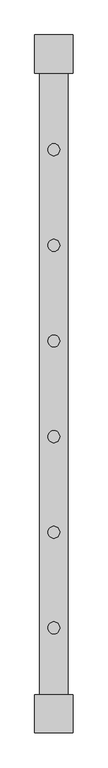
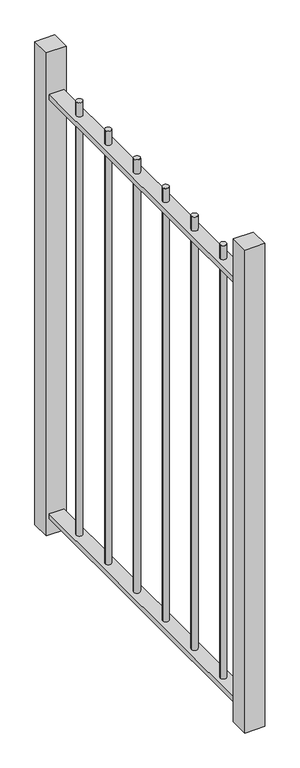
"""IFC4 building model written with IfcOpenShell, lengths in millimetres: railing geometry."""

from ifc_helpers import new_model, si_unit, point, frame, frame_2d, origin, place, context, project, spatial, polyline, circle_curve, trimmed, segment, composite_curve, outline, extrude, source, transform, mapped, element, save


def railing_e03dd60d(model_context):
    return source(origin(), model_context, "Body", "SweptSolid", [
        extrude(outline(polyline([(-6549.419961, 43748.8880881), (-6489.419961, 43748.8880881), (-6489.419961, 42369.1713717), (-6549.419961, 42369.1713717), (-6549.419961, 43748.8880881)])), frame((0.0, 0.0, -30.0), z_axis=(0.0, 0.0, 1.0), x_axis=(1.0, 0.0, 0.0)), (0.0, 0.0, 1.0), 20.0),
        extrude(outline(polyline([(-6549.419961, 43748.8880881), (-6489.419961, 43748.8880881), (-6489.419961, 42369.1713717), (-6549.419961, 42369.1713717), (-6549.419961, 43748.8880881)])), frame((0.0, 0.0, 1750.0), z_axis=(0.0, 0.0, 1.0), x_axis=(1.0, 0.0, 0.0)), (0.0, 0.0, 1.0), 20.0),
        extrude(outline(composite_curve([segment(trimmed(circle_curve(frame_2d((-6519.419961, 42548.8880881)), 12.5), [point((-6531.919961, 42548.8880881))], [point((-6506.919961, 42548.8880881))], False, "CARTESIAN"), True, "CONTINUOUS"), segment(trimmed(circle_curve(frame_2d((-6519.419961, 42548.8880881)), 12.5), [point((-6506.919961, 42548.8880881))], [point((-6531.919961, 42548.8880881))], False, "CARTESIAN"), True, "CONTINUOUS")], self_intersect=False)), frame((0.0, 0.0, -10.0), z_axis=(0.0, 0.0, 1.0), x_axis=(1.0, 0.0, 0.0)), (0.0, 0.0, 1.0), 1840.0),
        extrude(outline(composite_curve([segment(trimmed(circle_curve(frame_2d((-6519.419961, 42748.8880881)), 12.5), [point((-6531.919961, 42748.8880881))], [point((-6506.919961, 42748.8880881))], False, "CARTESIAN"), True, "CONTINUOUS"), segment(trimmed(circle_curve(frame_2d((-6519.419961, 42748.8880881)), 12.5), [point((-6506.919961, 42748.8880881))], [point((-6531.919961, 42748.8880881))], False, "CARTESIAN"), True, "CONTINUOUS")], self_intersect=False)), frame((0.0, 0.0, -10.0), z_axis=(0.0, 0.0, 1.0), x_axis=(1.0, 0.0, 0.0)), (0.0, 0.0, 1.0), 1840.0),
        extrude(outline(composite_curve([segment(trimmed(circle_curve(frame_2d((-6519.419961, 42948.8880881)), 12.5), [point((-6531.919961, 42948.8880881))], [point((-6506.919961, 42948.8880881))], False, "CARTESIAN"), True, "CONTINUOUS"), segment(trimmed(circle_curve(frame_2d((-6519.419961, 42948.8880881)), 12.5), [point((-6506.919961, 42948.8880881))], [point((-6531.919961, 42948.8880881))], False, "CARTESIAN"), True, "CONTINUOUS")], self_intersect=False)), frame((0.0, 0.0, -10.0), z_axis=(0.0, 0.0, 1.0), x_axis=(1.0, 0.0, 0.0)), (0.0, 0.0, 1.0), 1840.0),
        extrude(outline(composite_curve([segment(trimmed(circle_curve(frame_2d((-6519.419961, 43148.8880881)), 12.5), [point((-6531.919961, 43148.8880881))], [point((-6506.919961, 43148.8880881))], False, "CARTESIAN"), True, "CONTINUOUS"), segment(trimmed(circle_curve(frame_2d((-6519.419961, 43148.8880881)), 12.5), [point((-6506.919961, 43148.8880881))], [point((-6531.919961, 43148.8880881))], False, "CARTESIAN"), True, "CONTINUOUS")], self_intersect=False)), frame((0.0, 0.0, -10.0), z_axis=(0.0, 0.0, 1.0), x_axis=(1.0, 0.0, 0.0)), (0.0, 0.0, 1.0), 1840.0),
        extrude(outline(composite_curve([segment(trimmed(circle_curve(frame_2d((-6519.419961, 43348.8880881)), 12.5), [point((-6531.919961, 43348.8880881))], [point((-6506.919961, 43348.8880881))], False, "CARTESIAN"), True, "CONTINUOUS"), segment(trimmed(circle_curve(frame_2d((-6519.419961, 43348.8880881)), 12.5), [point((-6506.919961, 43348.8880881))], [point((-6531.919961, 43348.8880881))], False, "CARTESIAN"), True, "CONTINUOUS")], self_intersect=False)), frame((0.0, 0.0, -10.0), z_axis=(0.0, 0.0, 1.0), x_axis=(1.0, 0.0, 0.0)), (0.0, 0.0, 1.0), 1840.0),
        extrude(outline(composite_curve([segment(trimmed(circle_curve(frame_2d((-6519.419961, 43548.8880881)), 12.5), [point((-6531.919961, 43548.8880881))], [point((-6506.919961, 43548.8880881))], False, "CARTESIAN"), True, "CONTINUOUS"), segment(trimmed(circle_curve(frame_2d((-6519.419961, 43548.8880881)), 12.5), [point((-6506.919961, 43548.8880881))], [point((-6531.919961, 43548.8880881))], False, "CARTESIAN"), True, "CONTINUOUS")], self_intersect=False)), frame((0.0, 0.0, -10.0), z_axis=(0.0, 0.0, 1.0), x_axis=(1.0, 0.0, 0.0)), (0.0, 0.0, 1.0), 1840.0),
        extrude(outline(polyline([(-6479.419961, 42409.1713717), (-6479.419961, 42329.1713717), (-6559.419961, 42329.1713717), (-6559.419961, 42409.1713717), (-6479.419961, 42409.1713717)])), frame((0.0, 0.0, -100.0), z_axis=(0.0, 0.0, 1.0), x_axis=(1.0, 0.0, 0.0)), (0.0, 0.0, 1.0), 2050.0),
        extrude(outline(polyline([(-6479.419961, 43788.8880881), (-6479.419961, 43708.8880881), (-6559.419961, 43708.8880881), (-6559.419961, 43788.8880881), (-6479.419961, 43788.8880881)])), frame((0.0, 0.0, -100.0), z_axis=(0.0, 0.0, 1.0), x_axis=(1.0, 0.0, 0.0)), (0.0, 0.0, 1.0), 2050.0),
    ])


if __name__ == "__main__":
    model = new_model("IFC4")
    model_context = context("Model", 3, world=origin())
    ifc_project = project(units=[si_unit("LENGTHUNIT", "METRE", prefix="MILLI")], contexts=[model_context])
    site = spatial("IfcSite", under=ifc_project)
    building = spatial("IfcBuilding", under=site)
    placement = place(None, origin())
    railing_shape = railing_e03dd60d(model_context)
    element("IfcRailing", 1, at=placement, inside=building, context=model_context, shape_type="MappedRepresentation", body=[
        mapped(railing_shape, transform((0.0, 0.0, 0.0), x_axis=(1.0, 0.0, 0.0), y_axis=(0.0, 1.0, 0.0), z_axis=(0.0, 0.0, 1.0))),
    ])
    save(model, "model.ifc")

# Revit data of these elements
# Element 1 (IfcRailing)
#   Materials on its faces: "NLRS_h2_staal_generiek zwart_gen_rsf", "NLRS_h2_staal_gen_rsf"
# Materials
#   "NLRS_h2_staal_generiek zwart_gen_rsf": class "Metal", colour RGB 189 187 185, transparency 0, Manufacturer = "RevitGG", URL = "www.revitgg.nl", Description = "Staal, generiek materiaal", Cost = 0
#   "NLRS_h2_staal_gen_rsf": class "H - Metaal", colour RGB 189 187 185, transparency 0, Keynote = "h2", Model = "generiek", Manufacturer = "Revit Standards Foundation", URL = "www.revitstandards.org", Description = "staal", Cost = 0
